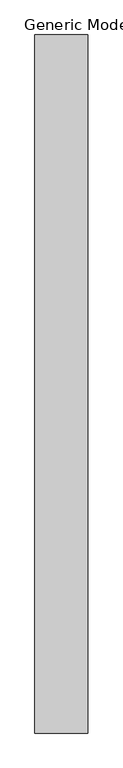
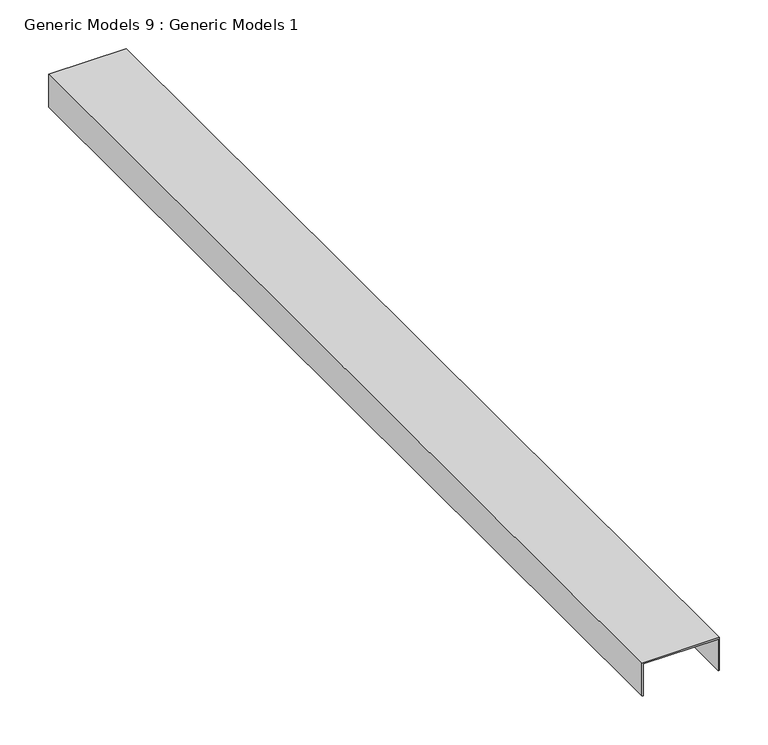
"""IFC4 building model written with IfcOpenShell, lengths in millimetres: proxy geometry, Generic Models 9 : Generic Models 1."""

from ifc_helpers import new_model, si_unit, frame, origin, place, context, project, spatial, polyline, outline, extrude, source, transform, mapped, element, save


def generic_models_9_generic_models_1_a88002d3(model_context):
    return source(origin(), model_context, "Body", "SweptSolid", [
        extrude(outline(polyline([(393.2679367, 51003.2), (393.2679367, 50911.125), (351.9929367, 50911.125), (351.9929367, 50912.7125), (391.6804367, 50912.7125), (391.6804367, 51001.6125), (351.9929367, 51001.6125), (351.9929367, 51003.2), (393.2679367, 51003.2)])), frame((0.0, 0.0, 0.0), z_axis=(0.0, 1.0, 0.0), x_axis=(0.0, 0.0, 1.0)), (0.0, 0.0, 1.0), 1219.2),
    ])


if __name__ == "__main__":
    model = new_model("IFC4")
    model_context = context("Model", 3, world=origin())
    ifc_project = project(units=[si_unit("LENGTHUNIT", "METRE", prefix="MILLI")], contexts=[model_context])
    site = spatial("IfcSite", under=ifc_project)
    building = spatial("IfcBuilding", under=site)
    placement = place(None, origin())
    generic_models_9_generic_models_1_shape = generic_models_9_generic_models_1_a88002d3(model_context)
    element("IfcBuildingElementProxy", 1, Name="Generic Models 9 : Generic Models 1", ObjectType="Generic Models 9 : Generic Models 1", at=placement, inside=building, context=model_context, shape_type="MappedRepresentation", body=[
        mapped(generic_models_9_generic_models_1_shape, transform((0.0, 0.0, 0.0), x_axis=(1.0, 0.0, 0.0), y_axis=(0.0, 1.0, 0.0), z_axis=(0.0, 0.0, 1.0))),
    ])
    save(model, "model.ifc")

# Revit data of these elements
# Element 1 (IfcBuildingElementProxy, "Generic Models 9 : Generic Models 1")
#   Materials on its faces: "METAL RUNNER ANCHORED TO STRUCTURE"
# Materials
#   "METAL RUNNER ANCHORED TO STRUCTURE": class "Unassigned", colour RGB 210 209 208, transparency 0, Keynote = "M05121300.02", Cost = 0
